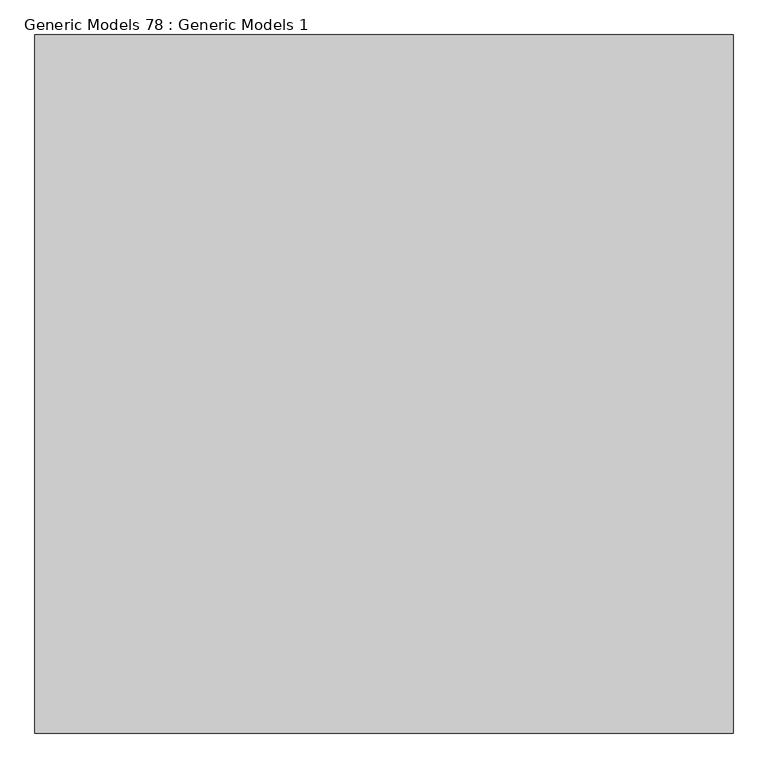
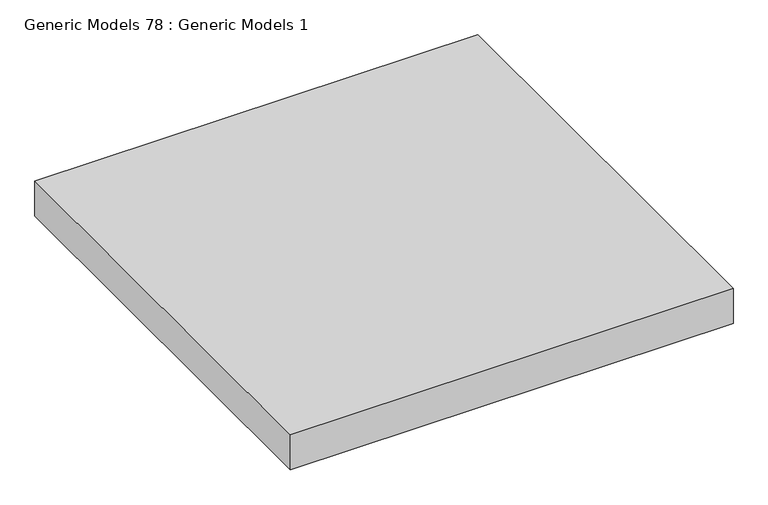
"""IFC4 building model written with IfcOpenShell, lengths in millimetres: proxy geometry, Generic Models 78 : Generic Models 1."""

from ifc_helpers import new_model, si_unit, frame, origin, place, context, project, spatial, polyline, outline, extrude, source, transform, mapped, element, save


def generic_models_78_generic_models_1_faebf22d(model_context):
    return source(origin(), model_context, "Body", "SweptSolid", [
        extrude(outline(polyline([(51649.6572697, 0.0), (50430.4572697, 0.0), (50430.4572697, 1219.2), (51649.6572697, 1219.2), (51649.6572697, 0.0)])), frame((0.0, 0.0, -73.749588), z_axis=(0.0, 0.0, 1.0), x_axis=(1.0, 0.0, 0.0)), (0.0, 0.0, 1.0), 101.6),
    ])


if __name__ == "__main__":
    model = new_model("IFC4")
    model_context = context("Model", 3, world=origin())
    ifc_project = project(units=[si_unit("LENGTHUNIT", "METRE", prefix="MILLI")], contexts=[model_context])
    site = spatial("IfcSite", under=ifc_project)
    building = spatial("IfcBuilding", under=site)
    placement = place(None, origin())
    generic_models_78_generic_models_1_shape = generic_models_78_generic_models_1_faebf22d(model_context)
    element("IfcBuildingElementProxy", 1, Name="Generic Models 78 : Generic Models 1", ObjectType="Generic Models 78 : Generic Models 1", at=placement, inside=building, context=model_context, shape_type="MappedRepresentation", body=[
        mapped(generic_models_78_generic_models_1_shape, transform((0.0, 0.0, 0.0), x_axis=(1.0, 0.0, 0.0), y_axis=(0.0, 1.0, 0.0), z_axis=(0.0, 0.0, 1.0))),
    ])
    save(model, "model.ifc")

# Revit data of these elements
# Element 1 (IfcBuildingElementProxy, "Generic Models 78 : Generic Models 1")
#   Materials on its faces: "STRUCTURAL FLOOR"
# Materials
#   "STRUCTURAL FLOOR": class "Concrete", colour RGB 115 116 108, transparency 0, Description = "Lightweight concrete", Cost = 0
